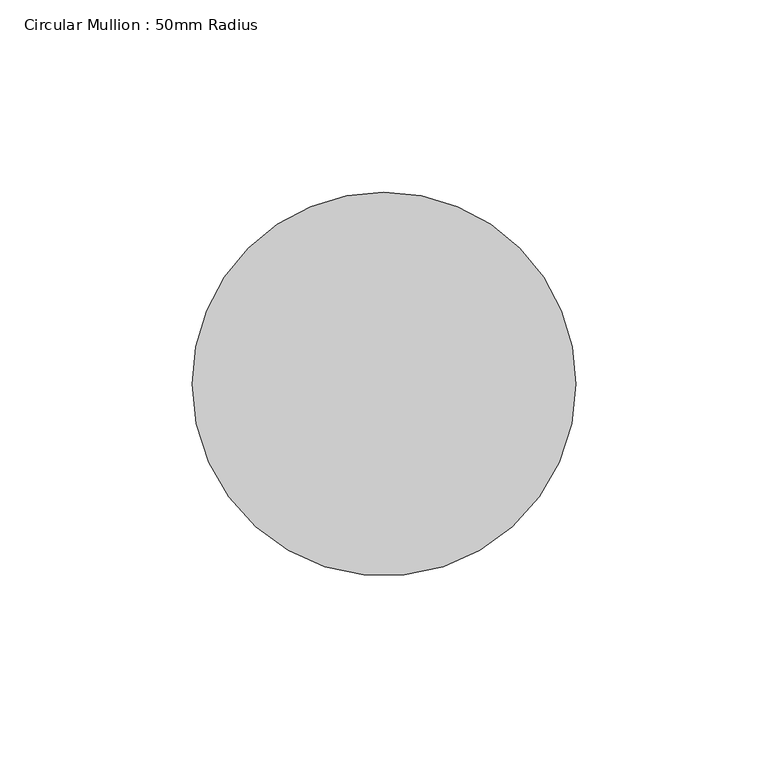
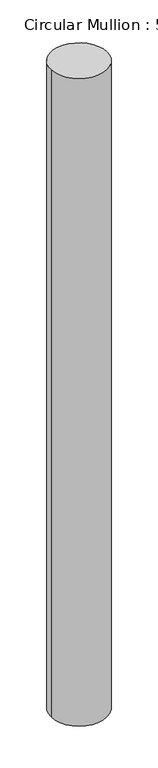
"""IFC4 building model written with IfcOpenShell, lengths in millimetres: member geometry, Circular Mullion : 50mm Radius."""

from ifc_helpers import new_model, si_unit, frame, origin, place, context, project, spatial, ellipse_curve, source, transform, mapped, element, save
from ifc_brep_helpers import plane_surface, cylinder_surface, advanced_brep


def circular_mullion_50mm_radius_a9279a7e(model_context):
    return source(origin(), model_context, "Body", "AdvancedBrep", [
        advanced_brep(
        [(-100.0, 0.0, 1.1891887), (0.0, 0.0, 0.0), (0.0, 0.0, -1221.7188054), (-100.0, 0.0, -1222.8394734)],
        [
            (0, 1, ellipse_curve(frame((-50.0, 0.0, 0.5945943), z_axis=(-0.011888858863068424, -0.01917979634234716, -0.9997453628035491), x_axis=(-0.5267218063576922, -0.8497381532886997, 0.02256567199974536)), 50.0127351, 50.0)),
            (1, 2),
            (2, 3, ellipse_curve(frame((-50.0, 0.0, -1222.2791394), z_axis=(-0.01120414534934138, -0.018075176807588227, 0.9997738519837202), x_axis=(0.5267368160521594, 0.8497623677979624, 0.021266050165326712)), 50.01131, 50.0)),
            (3, 0),
            (1, 0, ellipse_curve(frame((-50.0, 0.0, 0.5945943), z_axis=(-0.011888858863068424, -0.01917979634234716, -0.9997453628035491), x_axis=(-0.5267218063576922, -0.8497381532886997, 0.02256567199974536)), 50.0127351, 50.0)),
            (3, 2, ellipse_curve(frame((-50.0, 0.0, -1222.2791394), z_axis=(-0.01120414534934138, -0.018075176807588227, 0.9997738519837202), x_axis=(0.5267368160521594, 0.8497623677979624, 0.021266050165326712)), 50.01131, 50.0)),
        ],
        [
            cylinder_surface(frame((-50.0, 0.0, 0.0), z_axis=(0.0, 0.0, 1.0), x_axis=(1.0, 0.0, 0.0)), 50.0),
            plane_surface(frame((-259.066157, 160.5856977, 0.0), z_axis=(0.011888858863068428, 0.019179796342347163, 0.9997453628035493), x_axis=(0.5267218063576934, 0.8497381532886992, -0.022565671999740543))),
            plane_surface(frame((-259.066157, 160.5856977, -1221.7188054), z_axis=(0.01120414534934138, 0.018075176807588227, -0.9997738519837202), x_axis=(0.5267368160521593, 0.8497623677979621, 0.021266050165339667))),
        ],
        [
            (0, [[1, 2, 3, 4]]),
            (0, [[5, -4, 6, -2]]),
            (1, [[-1, -5]]),
            (2, [[-6, -3]]),
        ],
    ),
    ])


if __name__ == "__main__":
    model = new_model("IFC4")
    model_context = context("Model", 3, world=origin())
    ifc_project = project(units=[si_unit("LENGTHUNIT", "METRE", prefix="MILLI")], contexts=[model_context])
    site = spatial("IfcSite", under=ifc_project)
    building = spatial("IfcBuilding", under=site)
    placement = place(None, origin())
    circular_mullion_50mm_radius_shape = circular_mullion_50mm_radius_a9279a7e(model_context)
    element("IfcMember", 1, ObjectType="Circular Mullion : 50mm Radius", at=placement, inside=building, context=model_context, shape_type="MappedRepresentation", body=[
        mapped(circular_mullion_50mm_radius_shape, transform((0.0, 0.0, 0.0), x_axis=(1.0, 0.0, 0.0), y_axis=(0.0, 1.0, 0.0), z_axis=(0.0, 0.0, 1.0))),
    ])
    save(model, "model.ifc")

# Revit data of these elements
# Type "Circular Mullion : 50mm Radius"
#   built-in parameter 1007350 = 0.164042 (stored number, unit not read)
# Element 1 (IfcMember, "Circular Mullion : 50mm Radius")
#   Materials on its faces: "Aluminium"
# Materials
#   "Aluminium": class "Metal", colour RGB 247 247 247, transparency 0, Description = "Aluminium 6061", Cost = 0
